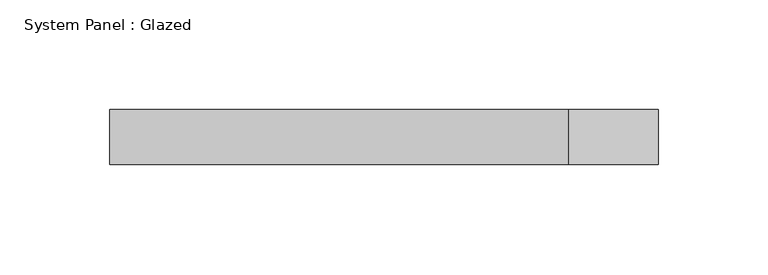
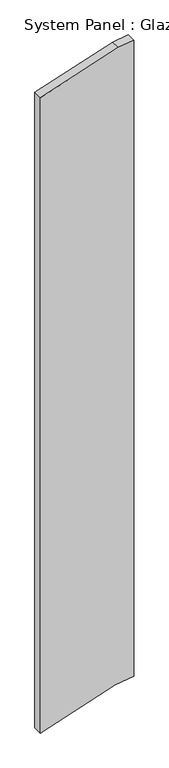
"""IFC4 building model written with IfcOpenShell, lengths in millimetres: plate geometry, System Panel : Glazed."""

from ifc_helpers import new_model, si_unit, frame, origin, place, context, project, spatial, polyline, outline, extrude, source, transform, mapped, element, save


def system_panel_glazed_8cec4914(model_context):
    return source(origin(), model_context, "Body", "SweptSolid", [
        extrude(outline(polyline([(0.0, -125.0), (66.2650818, 75.6194291), (73.361536, 125.0), (1874.3189879, 125.0), (1868.4480409, 84.1471034), (1799.3662478, -125.0), (0.0, -125.0)])), frame((0.0, 24.5, 0.0), z_axis=(0.0, 1.0, 0.0), x_axis=(0.0, 0.0, 1.0)), (0.0, 0.0, 1.0), 25.0),
    ])


if __name__ == "__main__":
    model = new_model("IFC4")
    model_context = context("Model", 3, world=origin())
    ifc_project = project(units=[si_unit("LENGTHUNIT", "METRE", prefix="MILLI")], contexts=[model_context])
    site = spatial("IfcSite", under=ifc_project)
    building = spatial("IfcBuilding", under=site)
    placement = place(None, origin())
    system_panel_glazed_shape = system_panel_glazed_8cec4914(model_context)
    element("IfcPlate", 1, ObjectType="System Panel : Glazed", at=placement, inside=building, context=model_context, shape_type="MappedRepresentation", body=[
        mapped(system_panel_glazed_shape, transform((0.0, 0.0, 0.0), x_axis=(1.0, 0.0, 0.0), y_axis=(0.0, 1.0, 0.0), z_axis=(0.0, 0.0, 1.0))),
    ])
    save(model, "model.ifc")

# Revit data of these elements
# Element 1 (IfcPlate, "System Panel : Glazed")
#   Materials on its faces: "Glass"
# Materials
#   "Glass": class "Glass", colour RGB 218 227 224, transparency 0.85, Description = "Soda Lime Glass", Cost = 0
